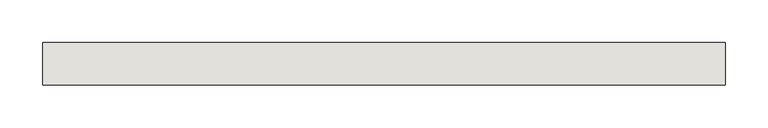
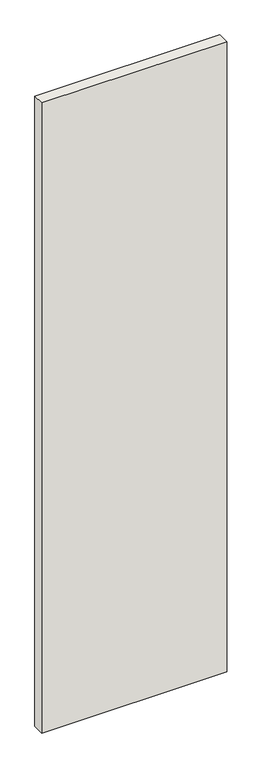
"""IFC4 building model written with IfcOpenShell, lengths in millimetres: wall geometry, 0_3d."""

from ifc_helpers import new_model, si_unit, origin, origin_with_axes, place, context, project, spatial, polyline, outline, extrude, source, transform, mapped, element, save


def wall_e83495ba(model_context):
    return source(origin(), model_context, "Body", "SweptSolid", [
        extrude(outline(polyline([(799.8390058, 50.0), (799.8390058, 0.0), (0.0, 0.0), (0.0, 50.0), (799.8390058, 50.0)])), origin_with_axes(), (0.0, 0.0, 1.0), 2880.0),
    ])


if __name__ == "__main__":
    model = new_model("IFC4")
    model_context = context("Model", 3, world=origin())
    ifc_project = project(units=[si_unit("LENGTHUNIT", "METRE", prefix="MILLI")], contexts=[model_context])
    site = spatial("IfcSite", under=ifc_project)
    building = spatial("IfcBuilding", under=site)
    placement = place(None, origin())
    wall_shape = wall_e83495ba(model_context)
    element("IfcWall", 1, ObjectType="0_3d", at=placement, inside=building, context=model_context, shape_type="MappedRepresentation", body=[
        mapped(wall_shape, transform((0.0, 0.0, 0.0), x_axis=(1.0, 0.0, 0.0), y_axis=(0.0, 1.0, 0.0), z_axis=(0.0, 0.0, 1.0))),
    ])
    save(model, "model.ifc")

# Revit data of these elements
# Element 1 (IfcWall, "0_3d")
#   Materials on its faces: "glas"
# Materials
#   "glas": class "Unassigned", colour RGB 250 253 254, transparency 0.95
